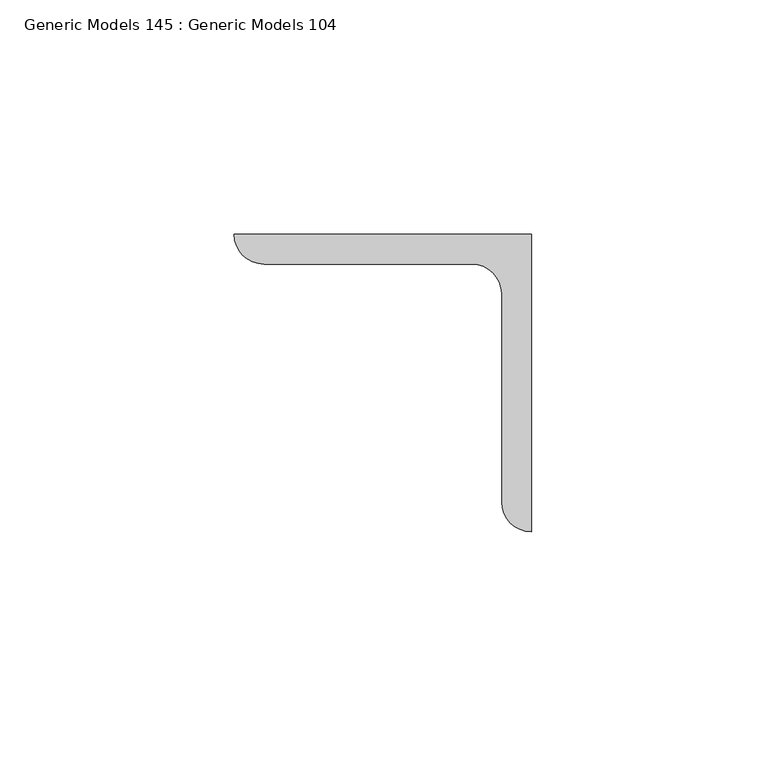
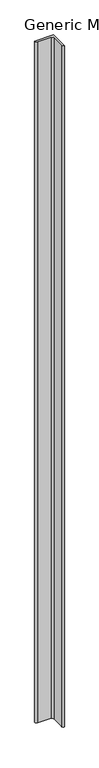
"""IFC4 building model written with IfcOpenShell, lengths in millimetres: proxy geometry, Generic Models 145 : Generic Models 104."""

from ifc_helpers import new_model, si_unit, point, frame, frame_2d, origin, place, context, project, spatial, polyline, circle_curve, trimmed, segment, composite_curve, outline, extrude, source, transform, mapped, element, save


def generic_models_145_generic_models_104_0ea7ce2d(model_context):
    return source(origin(), model_context, "Body", "SweptSolid", [
        extrude(outline(composite_curve([segment(polyline([(35362.35773, 41071.1196612), (35362.35773, 41007.6196612)]), True, "CONTINUOUS"), segment(trimmed(circle_curve(frame_2d((35362.35773, 41013.9696612)), 6.35), [point((35362.35773, 41007.6196612))], [point((35356.00773, 41013.9696612))], False, "CARTESIAN"), True, "CONTINUOUS"), segment(polyline([(35356.00773, 41013.9696612), (35356.00773, 41058.4196612)]), True, "CONTINUOUS"), segment(trimmed(circle_curve(frame_2d((35349.65773, 41058.4196612)), 6.35), [point((35356.00773, 41058.4196612))], [point((35349.65773, 41064.7696612))], True, "CARTESIAN"), True, "CONTINUOUS"), segment(polyline([(35349.65773, 41064.7696612), (35305.20773, 41064.7696612)]), True, "CONTINUOUS"), segment(trimmed(circle_curve(frame_2d((35305.20773, 41071.1196612)), 6.35), [point((35305.20773, 41064.7696612))], [point((35298.85773, 41071.1196612))], False, "CARTESIAN"), True, "CONTINUOUS"), segment(polyline([(35298.85773, 41071.1196612), (35362.35773, 41071.1196612)]), True, "CONTINUOUS")], self_intersect=False)), frame((0.0, 0.0, 266407.9), z_axis=(0.0, 0.0, 1.0), x_axis=(1.0, 0.0, 0.0)), (0.0, 0.0, 1.0), 2432.1044757),
    ])


if __name__ == "__main__":
    model = new_model("IFC4")
    model_context = context("Model", 3, world=origin())
    ifc_project = project(units=[si_unit("LENGTHUNIT", "METRE", prefix="MILLI")], contexts=[model_context])
    site = spatial("IfcSite", under=ifc_project)
    building = spatial("IfcBuilding", under=site)
    placement = place(None, origin())
    generic_models_145_generic_models_104_shape = generic_models_145_generic_models_104_0ea7ce2d(model_context)
    element("IfcBuildingElementProxy", 1, Name="Generic Models 145 : Generic Models 104", ObjectType="Generic Models 145 : Generic Models 104", at=placement, inside=building, context=model_context, shape_type="MappedRepresentation", body=[
        mapped(generic_models_145_generic_models_104_shape, transform((0.0, 0.0, 0.0), x_axis=(1.0, 0.0, 0.0), y_axis=(0.0, 1.0, 0.0), z_axis=(0.0, 0.0, 1.0))),
    ])
    save(model, "model.ifc")

# Revit data of these elements
# Element 1 (IfcBuildingElementProxy, "Generic Models 145 : Generic Models 104")
#   Materials on its faces: "(2) BACK/BACK GALVANIZED ANGLES (2) L2 1/2 X 2 1/2 X 1/4\")"
# Materials
#   "(2) BACK/BACK GALVANIZED ANGLES (2) L2 1/2 X 2 1/2 X 1/4\")": class "Unassigned", colour RGB 211 211 211, transparency 0, Cost = 0
